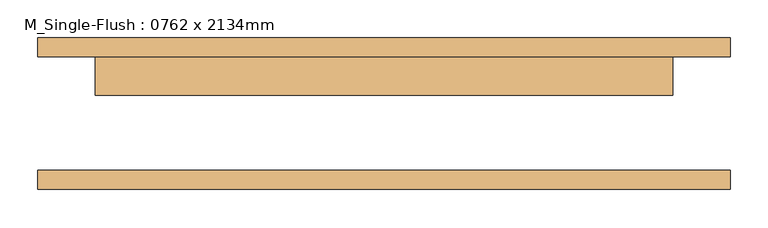
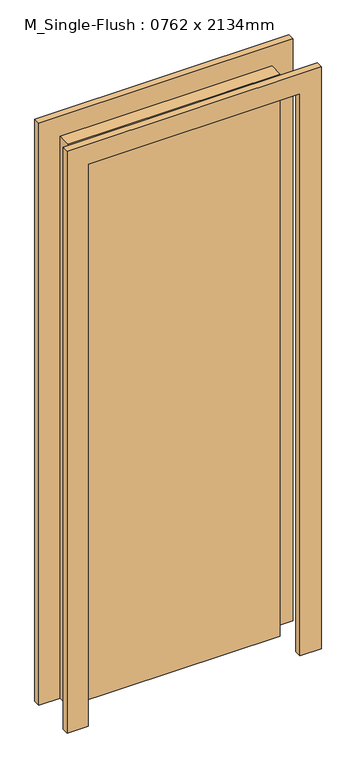
"""IFC4 building model written with IfcOpenShell, lengths in millimetres: door geometry, M_Single-Flush : 0762 x 2134mm."""

import ifcopenshell
import ifcopenshell.guid

model = None  # the IFC model being written
_history = None  # IfcOwnerHistory: only IFC2X3 demands one
_inside = {}  # id of a spatial element -> (the spatial element, [elements in it])
_under = {}  # id of a project, library or spatial element -> (it, [spatial elements below it])
_declared = {}  # id of a project -> (the project, [libraries it declares])
_typed = {}  # id of a type object -> (the type object, [elements of that type])
_made_of = {}  # id of a material, layer set ... -> (it, [elements and type objects made of it])


def new_model(schema):
    """Start an empty IFC model of exactly this schema.

    Asked for "IFC4X3", IfcOpenShell would pick the latest addendum, in which some entities
    have other attributes; the version numbers below select the first issue.
    IFC2X3 requires an IfcOwnerHistory on every rooted entity: one is made here for all.
    """
    global model, _history
    if schema == "IFC4X3":
        model = ifcopenshell.file(schema_version=(4, 3, 0, 0))
    else:
        model = ifcopenshell.file(schema=schema)
    _inside.clear()
    _under.clear()
    _declared.clear()
    _typed.clear()
    _made_of.clear()
    _history = None
    if model.schema == "IFC2X3":
        org = make("IfcOrganization", Name="unknown")
        user = make(
            "IfcPersonAndOrganization",
            ThePerson=make("IfcPerson", FamilyName="unknown"),
            TheOrganization=org,
        )
        app = make(
            "IfcApplication",
            ApplicationDeveloper=org,
            Version="unknown",
            ApplicationFullName="unknown",
            ApplicationIdentifier="unknown",
        )
        _history = make(
            "IfcOwnerHistory",
            OwningUser=user,
            OwningApplication=app,
            ChangeAction="ADDED",
            CreationDate=0,
        )
    return model


def make(cls, **values):
    """One entity of the class cls with the attributes given. An attribute that is None is left unset."""
    return model.create_entity(
        cls, **{name: value for name, value in values.items() if value is not None}
    )


def rooted(cls, **values):
    """An entity with a GlobalId (a new one), such as an element, a storey or a relation."""
    return make(cls, GlobalId=ifcopenshell.guid.new(), OwnerHistory=_history, **values)


def si_unit(unit_type, name, prefix=None):
    """IfcSIUnit, for example si_unit("LENGTHUNIT", "METRE", prefix="MILLI")."""
    return make("IfcSIUnit", UnitType=unit_type, Prefix=prefix, Name=name)


def assignment(units):
    """IfcUnitAssignment: the units of a project."""
    return None if units is None else make("IfcUnitAssignment", Units=units)


def point(xyz):
    """IfcCartesianPoint."""
    return None if xyz is None else make("IfcCartesianPoint", Coordinates=xyz)


def direction(xyz):
    """IfcDirection."""
    return None if xyz is None else make("IfcDirection", DirectionRatios=xyz)


def frame(location, z_axis=None, x_axis=None):
    """IfcAxis2Placement3D, a coordinate frame: its origin and axes. An axis left out is left unset."""
    return make(
        "IfcAxis2Placement3D",
        Location=point(location),
        Axis=direction(z_axis),
        RefDirection=direction(x_axis),
    )


def origin():
    """The frame at (0, 0, 0) with its axes left unset."""
    return frame((0.0, 0.0, 0.0))


def origin_with_axes():
    """The frame at (0, 0, 0) with the z axis (0, 0, 1) and the x axis (1, 0, 0) written out."""
    return frame((0.0, 0.0, 0.0), z_axis=(0.0, 0.0, 1.0), x_axis=(1.0, 0.0, 0.0))


def place(relative_to, where):
    """IfcLocalPlacement: puts the frame where relative to a parent placement (None: the world)."""
    return make(
        "IfcLocalPlacement", PlacementRelTo=relative_to, RelativePlacement=where
    )


def context(
    kind, dimensions, precision=None, world=None, true_north=None, identifier=None
):
    """IfcGeometricRepresentationContext, for example the 3D "Model" context."""
    return make(
        "IfcGeometricRepresentationContext",
        ContextIdentifier=identifier,
        ContextType=kind,
        CoordinateSpaceDimension=dimensions,
        Precision=precision,
        WorldCoordinateSystem=world,
        TrueNorth=true_north,
    )


def project(units=None, contexts=None):
    """IfcProject with its units and contexts."""
    return rooted(
        "IfcProject",
        Name="project",
        RepresentationContexts=contexts,
        UnitsInContext=assignment(units),
    )


def spatial(cls, under=None, at=None, **own):
    """A site, building, storey or space (cls), placed at a placement, below another one or the project."""
    s = rooted(cls, ObjectPlacement=at, **own)
    if under is not None:
        _under.setdefault(under.id(), (under, []))[1].append(s)
    return s


def polyline(points):
    """IfcPolyline through the points."""
    return make("IfcPolyline", Points=[point(p) for p in points])


def outline(outer, holes=None, kind="AREA"):
    """IfcArbitraryClosedProfileDef: a profile drawn as a closed curve; with holes, ...WithVoids."""
    if holes is None:
        return make("IfcArbitraryClosedProfileDef", ProfileType=kind, OuterCurve=outer)
    return make(
        "IfcArbitraryProfileDefWithVoids",
        ProfileType=kind,
        OuterCurve=outer,
        InnerCurves=holes,
    )


def extrude(swept, where, along, depth):
    """IfcExtrudedAreaSolid: the profile swept, set in the frame where, extruded along a direction by depth."""
    return make(
        "IfcExtrudedAreaSolid",
        SweptArea=swept,
        Position=where,
        ExtrudedDirection=direction(along),
        Depth=depth,
    )


def shape(context_of_items, identifier, shape_type, items):
    """IfcShapeRepresentation: the items that make up one representation, for example the "Body"."""
    return make(
        "IfcShapeRepresentation",
        ContextOfItems=context_of_items,
        RepresentationIdentifier=identifier,
        RepresentationType=shape_type,
        Items=items,
    )


def source(mapping_origin, context_of_items, identifier, shape_type, items):
    """IfcRepresentationMap: a shape defined once, which mapped items show again and again."""
    return make(
        "IfcRepresentationMap",
        MappingOrigin=mapping_origin,
        MappedRepresentation=shape(context_of_items, identifier, shape_type, items),
    )


def transform(
    local_origin,
    x_axis=None,
    y_axis=None,
    z_axis=None,
    scale=None,
    scale2=None,
    scale3=None,
    uniform=True,
):
    """IfcCartesianTransformationOperator3D, or its non-uniform kind. x_axis, y_axis, z_axis: its Axis1, 2, 3."""
    if uniform:
        return make(
            "IfcCartesianTransformationOperator3D",
            Axis1=direction(x_axis),
            Axis2=direction(y_axis),
            LocalOrigin=point(local_origin),
            Scale=scale,
            Axis3=direction(z_axis),
        )
    return make(
        "IfcCartesianTransformationOperator3DnonUniform",
        Axis1=direction(x_axis),
        Axis2=direction(y_axis),
        LocalOrigin=point(local_origin),
        Scale=scale,
        Axis3=direction(z_axis),
        Scale2=scale2,
        Scale3=scale3,
    )


def mapped(mapping_source, mapping_target):
    """IfcMappedItem: shows the shape of a source again, moved by a transform."""
    return make(
        "IfcMappedItem", MappingSource=mapping_source, MappingTarget=mapping_target
    )


def made_of(thing, what):
    """Note that an element or type object is made of a material, layer set ...; save() writes the relation."""
    if what is not None:
        _made_of.setdefault(what.id(), (what, []))[1].append(thing)
    return thing


def element(
    cls,
    number,
    at=None,
    inside=None,
    cuts=None,
    type_object=None,
    material=None,
    context=None,
    identifier="Body",
    shape_type=None,
    held_by="IfcProductDefinitionShape",
    body=None,
    shapes=None,
    **own,
):
    """One element of the class cls, such as IfcWall. Its Tag is "e" and its number.

    at: its placement. inside: the storey or other place that contains it. cuts: it is an
    opening in that element (IfcRelVoidsElement). A single representation is given by context,
    identifier, shape_type and body (its items); several are given by shapes. held_by: the class
    of the entity that holds the representations. save() writes the other relations.
    """
    e = rooted(cls, Tag="e%d" % number, ObjectPlacement=at, **own)
    if body is not None:
        shapes = [shape(context, identifier, shape_type, body)]
    if shapes is not None:
        e.Representation = make(held_by, Representations=shapes)
    if inside is not None:
        _inside.setdefault(inside.id(), (inside, []))[1].append(e)
    if cuts is not None:
        rooted(
            "IfcRelVoidsElement", RelatingBuildingElement=cuts, RelatedOpeningElement=e
        )
    if type_object is not None:
        _typed.setdefault(type_object.id(), (type_object, []))[1].append(e)
    return made_of(e, material)


def aggregate(whole, parts):
    """IfcRelAggregates: a whole, such as a stair, and the parts it consists of."""
    return rooted("IfcRelAggregates", RelatingObject=whole, RelatedObjects=parts)


def save(model, path):
    """Write the relations noted so far, then the file.

    IfcRelAggregates (storeys below a building ...), IfcRelContainedInSpatialStructure (elements
    in a storey), IfcRelDefinesByType, IfcRelAssociatesMaterial and IfcRelDeclares: one each for
    every whole, place, type object, material and project.
    """
    for whole, parts in _under.values():
        aggregate(whole, parts)
    for where, things in _inside.values():
        rooted(
            "IfcRelContainedInSpatialStructure",
            RelatedElements=things,
            RelatingStructure=where,
        )
    for kind, things in _typed.values():
        rooted("IfcRelDefinesByType", RelatedObjects=things, RelatingType=kind)
    for what, things in _made_of.values():
        rooted("IfcRelAssociatesMaterial", RelatedObjects=things, RelatingMaterial=what)
    for by, libraries in _declared.values():
        rooted("IfcRelDeclares", RelatingContext=by, RelatedDefinitions=libraries)
    model.write(path)


def m_single_flush_0762_x_2134mm_1533e4c5(model_context):
    return source(origin(), model_context, "Body", "SweptSolid", [
        extrude(outline(polyline([(2210.0, -457.0), (0.0, -457.0), (0.0, -381.0), (2134.0, -381.0), (2134.0, 381.0), (0.0, 381.0), (0.0, 457.0), (2210.0, 457.0), (2210.0, -457.0)])), frame((0.0, 75.0, 0.0), z_axis=(0.0, 1.0, 0.0), x_axis=(0.0, 0.0, 1.0)), (0.0, 0.0, 1.0), 25.0),
        extrude(outline(polyline([(2210.0, 457.0), (2210.0, -457.0), (0.0, -457.0), (0.0, -381.0), (2134.0, -381.0), (2134.0, 381.0), (0.0, 381.0), (0.0, 457.0), (2210.0, 457.0)])), frame((0.0, -100.0, 0.0), z_axis=(0.0, 1.0, 0.0), x_axis=(0.0, 0.0, 1.0)), (0.0, 0.0, 1.0), 25.0),
        extrude(outline(polyline([(381.0, 24.0), (-381.0, 24.0), (-381.0, 75.0), (381.0, 75.0), (381.0, 24.0)])), origin_with_axes(), (0.0, 0.0, 1.0), 2134.0),
    ])


if __name__ == "__main__":
    model = new_model("IFC4")
    model_context = context("Model", 3, world=origin())
    ifc_project = project(units=[si_unit("LENGTHUNIT", "METRE", prefix="MILLI")], contexts=[model_context])
    site = spatial("IfcSite", under=ifc_project)
    building = spatial("IfcBuilding", under=site)
    placement = place(None, origin())
    m_single_flush_0762_x_2134mm_shape = m_single_flush_0762_x_2134mm_1533e4c5(model_context)
    element("IfcDoor", 1, ObjectType="M_Single-Flush : 0762 x 2134mm", at=placement, inside=building, context=model_context, shape_type="MappedRepresentation", body=[
        mapped(m_single_flush_0762_x_2134mm_shape, transform((0.0, 0.0, 0.0), x_axis=(1.0, 0.0, 0.0), y_axis=(0.0, 1.0, 0.0), z_axis=(0.0, 0.0, 1.0))),
    ])
    save(model, "model.ifc")

# Revit data of these elements
# Type "M_Single-Flush : 0762 x 2134mm"
#   Type Mark = "18"
#   Thickness = 0.051 m
#   Height = 2.134 m
#   Trim Projection Ext = 0.025 m
#   Trim Projection Int = 0.025 m
#   Trim Width = 0.076 m
#   Width = 0.762 m
#   Door Material = Door - Panel
#   Frame Material = Door - Frame
#   Function = (empty or 0)
#   Wall Closure = (empty or 0)
# Element 1 (IfcDoor, "M_Single-Flush : 0762 x 2134mm")
#   Materials on its faces: "Door - Frame", "Door - Panel"
# Materials
#   "Door - Panel": class "Wood", colour RGB 114 82 51, transparency 0
#   "Door - Frame": class "Miscellaneous", colour RGB 255 0 128, transparency 0, Cost = 0
